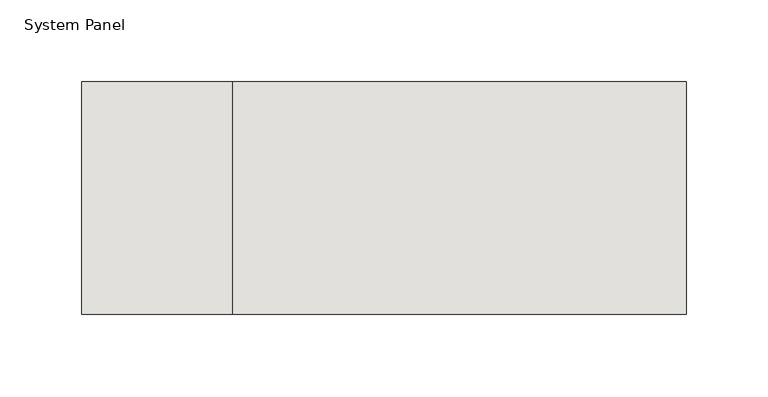
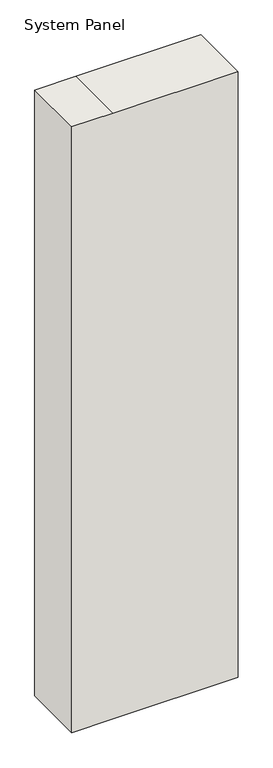
"""IFC4 building model written with IfcOpenShell, lengths in millimetres: wall geometry, System Panel : NLRS_21_CWP_hsb-vulling minerale wol 142 _gen_rsf."""

from ifc_helpers import new_model, si_unit, frame, origin, place, context, project, spatial, polyline, outline, extrude, source, transform, mapped, element, save


def system_panel_113e5983(model_context):
    return source(origin(), model_context, "Body", "SweptSolid", [
        extrude(outline(polyline([(0.0, -184.5), (0.0, -92.5), (0.0, 184.5), (1421.0, 184.5), (1421.0, -92.5), (1421.0, -184.5), (0.0, -184.5)])), frame((0.0, -71.0, 0.0), z_axis=(0.0, 1.0, 0.0), x_axis=(0.0, 0.0, 1.0)), (0.0, 0.0, 1.0), 142.0),
    ])


if __name__ == "__main__":
    model = new_model("IFC4")
    model_context = context("Model", 3, world=origin())
    ifc_project = project(units=[si_unit("LENGTHUNIT", "METRE", prefix="MILLI")], contexts=[model_context])
    site = spatial("IfcSite", under=ifc_project)
    building = spatial("IfcBuilding", under=site)
    placement = place(None, origin())
    system_panel_shape = system_panel_113e5983(model_context)
    element("IfcWall", 1, ObjectType="System Panel : NLRS_21_CWP_hsb-vulling minerale wol 142 _gen_rsf", at=placement, inside=building, context=model_context, shape_type="MappedRepresentation", body=[
        mapped(system_panel_shape, transform((0.0, 0.0, 0.0), x_axis=(1.0, 0.0, 0.0), y_axis=(0.0, 1.0, 0.0), z_axis=(0.0, 0.0, 1.0))),
    ])
    save(model, "model.ifc")

# Revit data of these elements
# Type "System Panel : NLRS_21_CWP_hsb-vulling minerale wol 142 _gen_rsf"
#   Type IfcGUID = "07M7mRoiH1CR8m_RSKIwpC"
#   Assembly Code = "21.23"
#   IfcExportAs = "IfcWall"
# Element 1 (IfcWall, "System Panel : NLRS_21_CWP_hsb-vulling minerale wol 142 _gen_rsf")
#   Materials on its faces: "NLRS_m1_isolatie minerale wol_gen_rsf"
# Materials
#   "NLRS_m1_isolatie minerale wol_gen_rsf": class "M - Anorganische materialen", colour RGB 200 200 140, transparency 0, Keynote = "m1", Manufacturer = "Revit Standards Foundation", URL = "www.revitstandards.org", Description = "isolatie minerale wol", Cost = 0
